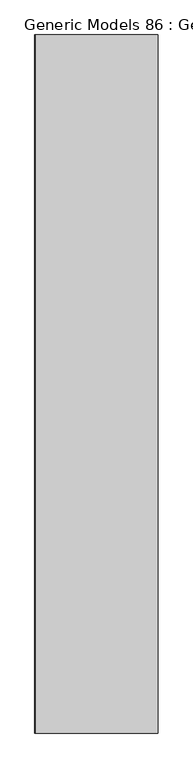
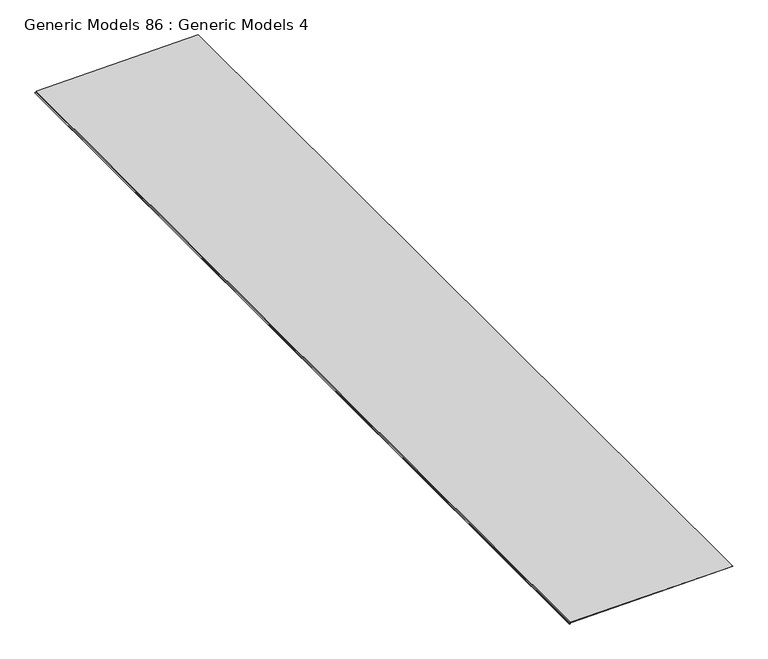
"""IFC4 building model written with IfcOpenShell, lengths in millimetres: proxy geometry, Generic Models 86 : Generic Models 4."""

from ifc_helpers import new_model, si_unit, frame, origin, place, context, project, spatial, polyline, outline, extrude, source, transform, mapped, element, save


def generic_models_86_generic_models_4_a0644872(model_context):
    return source(origin(), model_context, "Body", "SweptSolid", [
        extrude(outline(polyline([(126752.6729285, -5315.9872676), (126753.4665576, -5316.0011204), (126730.4892027, -6632.3729012), (126721.6749615, -6632.989253), (126721.6749615, -6643.2618229), (126720.8812115, -6643.2618229), (126720.8812115, -6632.2490691), (126729.7082674, -6631.6318212), (126752.6729285, -5315.9872676)])), frame((0.0, -464.1230338, 0.0), z_axis=(0.0, 1.0, 0.0), x_axis=(0.0, 0.0, 1.0)), (0.0, 0.0, 1.0), 7518.4),
    ])


if __name__ == "__main__":
    model = new_model("IFC4")
    model_context = context("Model", 3, world=origin())
    ifc_project = project(units=[si_unit("LENGTHUNIT", "METRE", prefix="MILLI")], contexts=[model_context])
    site = spatial("IfcSite", under=ifc_project)
    building = spatial("IfcBuilding", under=site)
    placement = place(None, origin())
    generic_models_86_generic_models_4_shape = generic_models_86_generic_models_4_a0644872(model_context)
    element("IfcBuildingElementProxy", 1, Name="Generic Models 86 : Generic Models 4", ObjectType="Generic Models 86 : Generic Models 4", at=placement, inside=building, context=model_context, shape_type="MappedRepresentation", body=[
        mapped(generic_models_86_generic_models_4_shape, transform((0.0, 0.0, 0.0), x_axis=(1.0, 0.0, 0.0), y_axis=(0.0, 1.0, 0.0), z_axis=(0.0, 0.0, 1.0))),
    ])
    save(model, "model.ifc")

# Revit data of these elements
# Element 1 (IfcBuildingElementProxy, "Generic Models 86 : Generic Models 4")
#   Materials on its faces: "_HYDROSTOP LIQUID MEMBRANE - FOLLOW MANU. RECOMMENDED INSTALLATION DETAILS"
# Materials
#   "_HYDROSTOP LIQUID MEMBRANE - FOLLOW MANU. RECOMMENDED INSTALLATION DETAILS": class "Generic", colour RGB 156 184 169, transparency 0, Cost = 0
